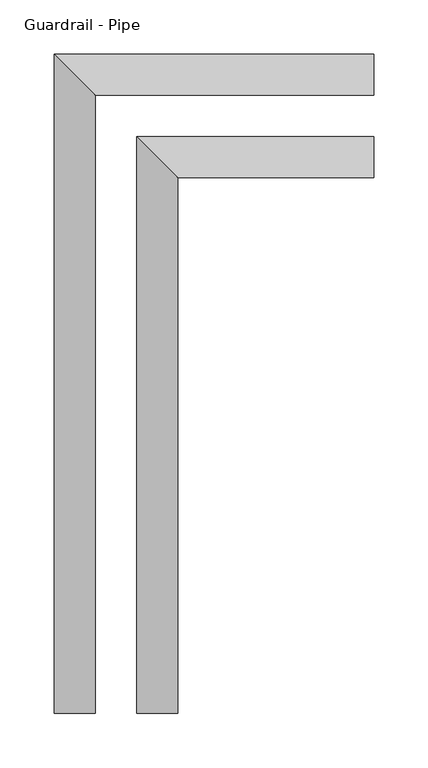
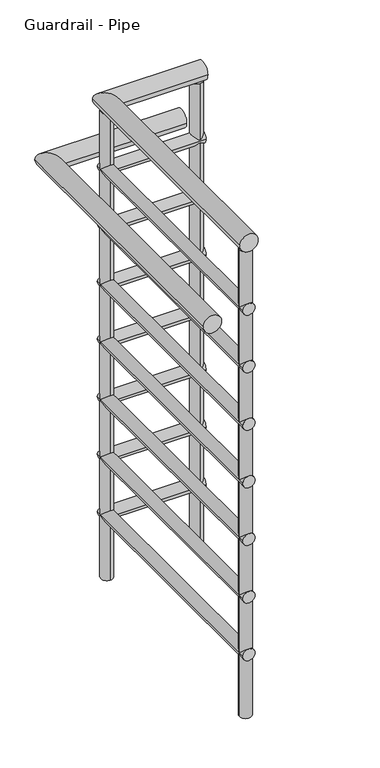
"""IFC4 building model written with IfcOpenShell, lengths in millimetres: railing geometry, Guardrail - Pipe."""

from ifc_helpers import new_model, si_unit, point, frame, frame_2d, origin, place, context, project, spatial, circle_curve, ellipse_curve, trimmed, segment, composite_curve, outline, extrude, source, transform, mapped, element, save
from ifc_brep_helpers import plane_surface, cylinder_surface, advanced_brep


def guardrail_pipe_7d06cf3b(model_context):
    return source(origin(), model_context, "Body", "SolidModel", [
        advanced_brep(
        [(-10864.1022358, -5457.4797826, 4705.35), (-10826.0022358, -5457.4797826, 4705.35), (-10864.1022358, -4924.0797826, 4705.35), (-10826.0022358, -4962.1797826, 4705.35), (-10645.1029016, -4924.0797826, 4705.35), (-10645.1029016, -4962.1797826, 4705.35)],
        [
            (0, 1, circle_curve(frame((-10845.0522358, -5457.4797826, 4705.35), z_axis=(0.0, -1.0, 0.0), x_axis=(1.0, 0.0, 0.0)), 19.05)),
            (1, 0, circle_curve(frame((-10845.0522358, -5457.4797826, 4705.35), z_axis=(0.0, -1.0, 0.0), x_axis=(1.0, 0.0, 0.0)), 19.05)),
            (2, 3, ellipse_curve(frame((-10845.0522358, -4943.1297826, 4705.35), z_axis=(-0.7071067811865502, -0.7071067811865449, 0.0), x_axis=(-0.707106781186545, 0.70710678118655, 0.0)), 26.9407684, 19.05)),
            (3, 1),
            (0, 2),
            (3, 2, ellipse_curve(frame((-10845.0522358, -4943.1297826, 4705.35), z_axis=(-0.7071067811865502, -0.7071067811865449, 0.0), x_axis=(-0.707106781186545, 0.70710678118655, 0.0)), 26.9407684, 19.05)),
            (4, 5, circle_curve(frame((-10645.1029016, -4943.1297826, 4705.35), z_axis=(1.0, 0.0, 0.0), x_axis=(0.0, -1.0, 0.0)), 19.05)),
            (5, 4, circle_curve(frame((-10645.1029016, -4943.1297826, 4705.35), z_axis=(1.0, 0.0, 0.0), x_axis=(0.0, -1.0, 0.0)), 19.05)),
            (5, 3),
            (2, 4),
        ],
        [
            plane_surface(frame((-10845.0522358, -5457.4797826, 4724.4), z_axis=(0.0, -1.0, 0.0), x_axis=(0.0, 0.0, -1.0))),
            cylinder_surface(frame((-10845.0522358, -4943.1297826, 4705.35), z_axis=(0.0, 1.0, 0.0), x_axis=(1.0, 0.0, 0.0)), 19.05),
            plane_surface(frame((-10645.1029016, -4943.1297826, 4724.4), z_axis=(1.0, 0.0, 0.0), x_axis=(0.0, -1.0, 0.0))),
            cylinder_surface(frame((-10645.1029016, -4943.1297826, 4705.35), z_axis=(1.0, 0.0, 0.0), x_axis=(0.0, -1.0, 0.0)), 19.05),
        ],
        [
            (0, [[1, 2]]),
            (1, [[3, 4, -1, 5]]),
            (1, [[6, -5, -2, -4]]),
            (2, [[7, 8]]),
            (3, [[-8, 9, -3, 10]]),
            (3, [[-7, -10, -6, -9]]),
        ],
    ),
        advanced_brep(
        [(-10645.1029016, -4930.4297826, 4559.3), (-10645.1029016, -4955.8297826, 4559.3), (-10832.3522358, -4955.8297826, 4559.3), (-10857.7522358, -4930.4297826, 4559.3), (-10857.7522358, -5457.4797826, 4559.3), (-10832.3522358, -5457.4797826, 4559.3)],
        [
            (0, 1, circle_curve(frame((-10645.1029016, -4943.1297826, 4559.3), z_axis=(1.0, 0.0, 0.0), x_axis=(0.0, -1.0, 0.0)), 12.7)),
            (1, 0, circle_curve(frame((-10645.1029016, -4943.1297826, 4559.3), z_axis=(1.0, 0.0, 0.0), x_axis=(0.0, -1.0, 0.0)), 12.7)),
            (1, 2),
            (2, 3, ellipse_curve(frame((-10845.0522358, -4943.1297826, 4559.3), z_axis=(0.7071067811865502, 0.7071067811865449, 0.0), x_axis=(0.7071067811865447, -0.7071067811865503, 0.0)), 17.9605122, 12.7)),
            (3, 0),
            (3, 2, ellipse_curve(frame((-10845.0522358, -4943.1297826, 4559.3), z_axis=(0.7071067811865502, 0.7071067811865449, 0.0), x_axis=(0.7071067811865447, -0.7071067811865503, 0.0)), 17.9605122, 12.7)),
            (4, 5, circle_curve(frame((-10845.0522358, -5457.4797826, 4559.3), z_axis=(0.0, -1.0, 0.0), x_axis=(1.0, 0.0, 0.0)), 12.7)),
            (5, 4, circle_curve(frame((-10845.0522358, -5457.4797826, 4559.3), z_axis=(0.0, -1.0, 0.0), x_axis=(1.0, 0.0, 0.0)), 12.7)),
            (2, 5),
            (4, 3),
        ],
        [
            plane_surface(frame((-10645.1029016, -4943.1297826, 4572.0), z_axis=(1.0, 0.0, 0.0), x_axis=(0.0, -1.0, 0.0))),
            cylinder_surface(frame((-10645.1029016, -4943.1297826, 4559.3), z_axis=(1.0, 0.0, 0.0), x_axis=(0.0, -1.0, 0.0)), 12.7),
            plane_surface(frame((-10845.0522358, -5457.4797826, 4572.0), z_axis=(0.0, -1.0, 0.0), x_axis=(0.0, 0.0, -1.0))),
            cylinder_surface(frame((-10845.0522358, -4943.1297826, 4559.3), z_axis=(0.0, 1.0, 0.0), x_axis=(1.0, 0.0, 0.0)), 12.7),
        ],
        [
            (0, [[1, 2]]),
            (1, [[-2, 3, 4, 5]]),
            (1, [[-1, -5, 6, -3]]),
            (2, [[7, 8]]),
            (3, [[-4, 9, -7, 10]]),
            (3, [[-6, -10, -8, -9]]),
        ],
    ),
        advanced_brep(
        [(-10940.3022358, -5457.4797826, 4552.95), (-10902.2022358, -5457.4797826, 4552.95), (-10940.3022358, -4847.8797826, 4552.95), (-10902.2022358, -4885.9797826, 4552.95), (-10645.1029016, -4847.8797826, 4552.95), (-10645.1029016, -4885.9797826, 4552.95)],
        [
            (0, 1, circle_curve(frame((-10921.2522358, -5457.4797826, 4552.95), z_axis=(0.0, -1.0, 0.0), x_axis=(1.0, 0.0, 0.0)), 19.05)),
            (1, 0, circle_curve(frame((-10921.2522358, -5457.4797826, 4552.95), z_axis=(0.0, -1.0, 0.0), x_axis=(1.0, 0.0, 0.0)), 19.05)),
            (2, 3, ellipse_curve(frame((-10921.2522358, -4866.9297826, 4552.95), z_axis=(-0.7071067811865502, -0.7071067811865449, 0.0), x_axis=(-0.707106781186545, 0.70710678118655, 0.0)), 26.9407684, 19.05)),
            (3, 1),
            (0, 2),
            (3, 2, ellipse_curve(frame((-10921.2522358, -4866.9297826, 4552.95), z_axis=(-0.7071067811865502, -0.7071067811865449, 0.0), x_axis=(-0.707106781186545, 0.70710678118655, 0.0)), 26.9407684, 19.05)),
            (4, 5, circle_curve(frame((-10645.1029016, -4866.9297826, 4552.95), z_axis=(1.0, 0.0, 0.0), x_axis=(0.0, -1.0, 0.0)), 19.05)),
            (5, 4, circle_curve(frame((-10645.1029016, -4866.9297826, 4552.95), z_axis=(1.0, 0.0, 0.0), x_axis=(0.0, -1.0, 0.0)), 19.05)),
            (4, 2),
            (3, 5),
        ],
        [
            plane_surface(frame((-10921.2522358, -5457.4797826, 4572.0), z_axis=(0.0, -1.0, 0.0), x_axis=(0.0, 0.0, -1.0))),
            cylinder_surface(frame((-10921.2522358, -4866.9297826, 4552.95), z_axis=(0.0, 1.0, 0.0), x_axis=(1.0, 0.0, 0.0)), 19.05),
            plane_surface(frame((-10645.1029016, -4866.9297826, 4572.0), z_axis=(1.0, 0.0, 0.0), x_axis=(0.0, -1.0, 0.0))),
            cylinder_surface(frame((-10645.1029016, -4866.9297826, 4552.95), z_axis=(1.0, 0.0, 0.0), x_axis=(0.0, -1.0, 0.0)), 19.05),
        ],
        [
            (0, [[1, 2]]),
            (1, [[3, 4, -1, 5]]),
            (1, [[6, -5, -2, -4]]),
            (2, [[7, 8]]),
            (3, [[-7, 9, -6, 10]]),
            (3, [[-8, -10, -3, -9]]),
        ],
    ),
        advanced_brep(
        [(-10645.1029016, -4930.4297826, 4432.3), (-10645.1029016, -4955.8297826, 4432.3), (-10832.3522358, -4955.8297826, 4432.3), (-10857.7522358, -4930.4297826, 4432.3), (-10857.7522358, -5457.4797826, 4432.3), (-10832.3522358, -5457.4797826, 4432.3)],
        [
            (0, 1, circle_curve(frame((-10645.1029016, -4943.1297826, 4432.3), z_axis=(1.0, 0.0, 0.0), x_axis=(0.0, -1.0, 0.0)), 12.7)),
            (1, 0, circle_curve(frame((-10645.1029016, -4943.1297826, 4432.3), z_axis=(1.0, 0.0, 0.0), x_axis=(0.0, -1.0, 0.0)), 12.7)),
            (1, 2),
            (2, 3, ellipse_curve(frame((-10845.0522358, -4943.1297826, 4432.3), z_axis=(0.7071067811865502, 0.7071067811865449, 0.0), x_axis=(0.7071067811865447, -0.7071067811865503, 0.0)), 17.9605122, 12.7)),
            (3, 0),
            (3, 2, ellipse_curve(frame((-10845.0522358, -4943.1297826, 4432.3), z_axis=(0.7071067811865502, 0.7071067811865449, 0.0), x_axis=(0.7071067811865447, -0.7071067811865503, 0.0)), 17.9605122, 12.7)),
            (4, 5, circle_curve(frame((-10845.0522358, -5457.4797826, 4432.3), z_axis=(0.0, -1.0, 0.0), x_axis=(1.0, 0.0, 0.0)), 12.7)),
            (5, 4, circle_curve(frame((-10845.0522358, -5457.4797826, 4432.3), z_axis=(0.0, -1.0, 0.0), x_axis=(1.0, 0.0, 0.0)), 12.7)),
            (2, 5),
            (4, 3),
        ],
        [
            plane_surface(frame((-10645.1029016, -4943.1297826, 4445.0), z_axis=(1.0, 0.0, 0.0), x_axis=(0.0, -1.0, 0.0))),
            cylinder_surface(frame((-10645.1029016, -4943.1297826, 4432.3), z_axis=(1.0, 0.0, 0.0), x_axis=(0.0, -1.0, 0.0)), 12.7),
            plane_surface(frame((-10845.0522358, -5457.4797826, 4445.0), z_axis=(0.0, -1.0, 0.0), x_axis=(0.0, 0.0, -1.0))),
            cylinder_surface(frame((-10845.0522358, -4943.1297826, 4432.3), z_axis=(0.0, 1.0, 0.0), x_axis=(1.0, 0.0, 0.0)), 12.7),
        ],
        [
            (0, [[1, 2]]),
            (1, [[-2, 3, 4, 5]]),
            (1, [[-1, -5, 6, -3]]),
            (2, [[7, 8]]),
            (3, [[-4, 9, -7, 10]]),
            (3, [[-6, -10, -8, -9]]),
        ],
    ),
        advanced_brep(
        [(-10645.1029016, -4930.4297826, 4305.3), (-10645.1029016, -4955.8297826, 4305.3), (-10832.3522358, -4955.8297826, 4305.3), (-10857.7522358, -4930.4297826, 4305.3), (-10857.7522358, -5457.4797826, 4305.3), (-10832.3522358, -5457.4797826, 4305.3)],
        [
            (0, 1, circle_curve(frame((-10645.1029016, -4943.1297826, 4305.3), z_axis=(1.0, 0.0, 0.0), x_axis=(0.0, -1.0, 0.0)), 12.7)),
            (1, 0, circle_curve(frame((-10645.1029016, -4943.1297826, 4305.3), z_axis=(1.0, 0.0, 0.0), x_axis=(0.0, -1.0, 0.0)), 12.7)),
            (1, 2),
            (2, 3, ellipse_curve(frame((-10845.0522358, -4943.1297826, 4305.3), z_axis=(0.7071067811865502, 0.7071067811865449, 0.0), x_axis=(0.7071067811865447, -0.7071067811865503, 0.0)), 17.9605122, 12.7)),
            (3, 0),
            (3, 2, ellipse_curve(frame((-10845.0522358, -4943.1297826, 4305.3), z_axis=(0.7071067811865502, 0.7071067811865449, 0.0), x_axis=(0.7071067811865447, -0.7071067811865503, 0.0)), 17.9605122, 12.7)),
            (4, 5, circle_curve(frame((-10845.0522358, -5457.4797826, 4305.3), z_axis=(0.0, -1.0, 0.0), x_axis=(1.0, 0.0, 0.0)), 12.7)),
            (5, 4, circle_curve(frame((-10845.0522358, -5457.4797826, 4305.3), z_axis=(0.0, -1.0, 0.0), x_axis=(1.0, 0.0, 0.0)), 12.7)),
            (2, 5),
            (4, 3),
        ],
        [
            plane_surface(frame((-10645.1029016, -4943.1297826, 4318.0), z_axis=(1.0, 0.0, 0.0), x_axis=(0.0, -1.0, 0.0))),
            cylinder_surface(frame((-10645.1029016, -4943.1297826, 4305.3), z_axis=(1.0, 0.0, 0.0), x_axis=(0.0, -1.0, 0.0)), 12.7),
            plane_surface(frame((-10845.0522358, -5457.4797826, 4318.0), z_axis=(0.0, -1.0, 0.0), x_axis=(0.0, 0.0, -1.0))),
            cylinder_surface(frame((-10845.0522358, -4943.1297826, 4305.3), z_axis=(0.0, 1.0, 0.0), x_axis=(1.0, 0.0, 0.0)), 12.7),
        ],
        [
            (0, [[1, 2]]),
            (1, [[-2, 3, 4, 5]]),
            (1, [[-1, -5, 6, -3]]),
            (2, [[7, 8]]),
            (3, [[-4, 9, -7, 10]]),
            (3, [[-6, -10, -8, -9]]),
        ],
    ),
        advanced_brep(
        [(-10645.1029016, -4930.4297826, 4178.3), (-10645.1029016, -4955.8297826, 4178.3), (-10832.3522358, -4955.8297826, 4178.3), (-10857.7522358, -4930.4297826, 4178.3), (-10857.7522358, -5457.4797826, 4178.3), (-10832.3522358, -5457.4797826, 4178.3)],
        [
            (0, 1, circle_curve(frame((-10645.1029016, -4943.1297826, 4178.3), z_axis=(1.0, 0.0, 0.0), x_axis=(0.0, -1.0, 0.0)), 12.7)),
            (1, 0, circle_curve(frame((-10645.1029016, -4943.1297826, 4178.3), z_axis=(1.0, 0.0, 0.0), x_axis=(0.0, -1.0, 0.0)), 12.7)),
            (1, 2),
            (2, 3, ellipse_curve(frame((-10845.0522358, -4943.1297826, 4178.3), z_axis=(0.7071067811865502, 0.7071067811865449, 0.0), x_axis=(0.7071067811865447, -0.7071067811865503, 0.0)), 17.9605122, 12.7)),
            (3, 0),
            (3, 2, ellipse_curve(frame((-10845.0522358, -4943.1297826, 4178.3), z_axis=(0.7071067811865502, 0.7071067811865449, 0.0), x_axis=(0.7071067811865447, -0.7071067811865503, 0.0)), 17.9605122, 12.7)),
            (4, 5, circle_curve(frame((-10845.0522358, -5457.4797826, 4178.3), z_axis=(0.0, -1.0, 0.0), x_axis=(1.0, 0.0, 0.0)), 12.7)),
            (5, 4, circle_curve(frame((-10845.0522358, -5457.4797826, 4178.3), z_axis=(0.0, -1.0, 0.0), x_axis=(1.0, 0.0, 0.0)), 12.7)),
            (2, 5),
            (4, 3),
        ],
        [
            plane_surface(frame((-10645.1029016, -4943.1297826, 4191.0), z_axis=(1.0, 0.0, 0.0), x_axis=(0.0, -1.0, 0.0))),
            cylinder_surface(frame((-10645.1029016, -4943.1297826, 4178.3), z_axis=(1.0, 0.0, 0.0), x_axis=(0.0, -1.0, 0.0)), 12.7),
            plane_surface(frame((-10845.0522358, -5457.4797826, 4191.0), z_axis=(0.0, -1.0, 0.0), x_axis=(0.0, 0.0, -1.0))),
            cylinder_surface(frame((-10845.0522358, -4943.1297826, 4178.3), z_axis=(0.0, 1.0, 0.0), x_axis=(1.0, 0.0, 0.0)), 12.7),
        ],
        [
            (0, [[1, 2]]),
            (1, [[-2, 3, 4, 5]]),
            (1, [[-1, -5, 6, -3]]),
            (2, [[7, 8]]),
            (3, [[-4, 9, -7, 10]]),
            (3, [[-6, -10, -8, -9]]),
        ],
    ),
        advanced_brep(
        [(-10645.1029016, -4930.4297826, 4051.3), (-10645.1029016, -4955.8297826, 4051.3), (-10832.3522358, -4955.8297826, 4051.3), (-10857.7522358, -4930.4297826, 4051.3), (-10857.7522358, -5457.4797826, 4051.3), (-10832.3522358, -5457.4797826, 4051.3)],
        [
            (0, 1, circle_curve(frame((-10645.1029016, -4943.1297826, 4051.3), z_axis=(1.0, 0.0, 0.0), x_axis=(0.0, -1.0, 0.0)), 12.7)),
            (1, 0, circle_curve(frame((-10645.1029016, -4943.1297826, 4051.3), z_axis=(1.0, 0.0, 0.0), x_axis=(0.0, -1.0, 0.0)), 12.7)),
            (1, 2),
            (2, 3, ellipse_curve(frame((-10845.0522358, -4943.1297826, 4051.3), z_axis=(0.7071067811865502, 0.7071067811865449, 0.0), x_axis=(0.7071067811865447, -0.7071067811865503, 0.0)), 17.9605122, 12.7)),
            (3, 0),
            (3, 2, ellipse_curve(frame((-10845.0522358, -4943.1297826, 4051.3), z_axis=(0.7071067811865502, 0.7071067811865449, 0.0), x_axis=(0.7071067811865447, -0.7071067811865503, 0.0)), 17.9605122, 12.7)),
            (4, 5, circle_curve(frame((-10845.0522358, -5457.4797826, 4051.3), z_axis=(0.0, -1.0, 0.0), x_axis=(1.0, 0.0, 0.0)), 12.7)),
            (5, 4, circle_curve(frame((-10845.0522358, -5457.4797826, 4051.3), z_axis=(0.0, -1.0, 0.0), x_axis=(1.0, 0.0, 0.0)), 12.7)),
            (2, 5),
            (4, 3),
        ],
        [
            plane_surface(frame((-10645.1029016, -4943.1297826, 4064.0), z_axis=(1.0, 0.0, 0.0), x_axis=(0.0, -1.0, 0.0))),
            cylinder_surface(frame((-10645.1029016, -4943.1297826, 4051.3), z_axis=(1.0, 0.0, 0.0), x_axis=(0.0, -1.0, 0.0)), 12.7),
            plane_surface(frame((-10845.0522358, -5457.4797826, 4064.0), z_axis=(0.0, -1.0, 0.0), x_axis=(0.0, 0.0, -1.0))),
            cylinder_surface(frame((-10845.0522358, -4943.1297826, 4051.3), z_axis=(0.0, 1.0, 0.0), x_axis=(1.0, 0.0, 0.0)), 12.7),
        ],
        [
            (0, [[1, 2]]),
            (1, [[-2, 3, 4, 5]]),
            (1, [[-1, -5, 6, -3]]),
            (2, [[7, 8]]),
            (3, [[-4, 9, -7, 10]]),
            (3, [[-6, -10, -8, -9]]),
        ],
    ),
        advanced_brep(
        [(-10645.1029016, -4930.4297826, 3924.3), (-10645.1029016, -4955.8297826, 3924.3), (-10832.3522358, -4955.8297826, 3924.3), (-10857.7522358, -4930.4297826, 3924.3), (-10857.7522358, -5457.4797826, 3924.3), (-10832.3522358, -5457.4797826, 3924.3)],
        [
            (0, 1, circle_curve(frame((-10645.1029016, -4943.1297826, 3924.3), z_axis=(1.0, 0.0, 0.0), x_axis=(0.0, -1.0, 0.0)), 12.7)),
            (1, 0, circle_curve(frame((-10645.1029016, -4943.1297826, 3924.3), z_axis=(1.0, 0.0, 0.0), x_axis=(0.0, -1.0, 0.0)), 12.7)),
            (1, 2),
            (2, 3, ellipse_curve(frame((-10845.0522358, -4943.1297826, 3924.3), z_axis=(0.7071067811865502, 0.7071067811865449, 0.0), x_axis=(0.7071067811865447, -0.7071067811865503, 0.0)), 17.9605122, 12.7)),
            (3, 0),
            (3, 2, ellipse_curve(frame((-10845.0522358, -4943.1297826, 3924.3), z_axis=(0.7071067811865502, 0.7071067811865449, 0.0), x_axis=(0.7071067811865447, -0.7071067811865503, 0.0)), 17.9605122, 12.7)),
            (4, 5, circle_curve(frame((-10845.0522358, -5457.4797826, 3924.3), z_axis=(0.0, -1.0, 0.0), x_axis=(1.0, 0.0, 0.0)), 12.7)),
            (5, 4, circle_curve(frame((-10845.0522358, -5457.4797826, 3924.3), z_axis=(0.0, -1.0, 0.0), x_axis=(1.0, 0.0, 0.0)), 12.7)),
            (2, 5),
            (4, 3),
        ],
        [
            plane_surface(frame((-10645.1029016, -4943.1297826, 3937.0), z_axis=(1.0, 0.0, 0.0), x_axis=(0.0, -1.0, 0.0))),
            cylinder_surface(frame((-10645.1029016, -4943.1297826, 3924.3), z_axis=(1.0, 0.0, 0.0), x_axis=(0.0, -1.0, 0.0)), 12.7),
            plane_surface(frame((-10845.0522358, -5457.4797826, 3937.0), z_axis=(0.0, -1.0, 0.0), x_axis=(0.0, 0.0, -1.0))),
            cylinder_surface(frame((-10845.0522358, -4943.1297826, 3924.3), z_axis=(0.0, 1.0, 0.0), x_axis=(1.0, 0.0, 0.0)), 12.7),
        ],
        [
            (0, [[1, 2]]),
            (1, [[-2, 3, 4, 5]]),
            (1, [[-1, -5, 6, -3]]),
            (2, [[7, 8]]),
            (3, [[-4, 9, -7, 10]]),
            (3, [[-6, -10, -8, -9]]),
        ],
    ),
        advanced_brep(
        [(-10645.1029016, -4930.4297826, 3797.3), (-10645.1029016, -4955.8297826, 3797.3), (-10832.3522358, -4955.8297826, 3797.3), (-10857.7522358, -4930.4297826, 3797.3), (-10857.7522358, -5457.4797826, 3797.3), (-10832.3522358, -5457.4797826, 3797.3)],
        [
            (0, 1, circle_curve(frame((-10645.1029016, -4943.1297826, 3797.3), z_axis=(1.0, 0.0, 0.0), x_axis=(0.0, -1.0, 0.0)), 12.7)),
            (1, 0, circle_curve(frame((-10645.1029016, -4943.1297826, 3797.3), z_axis=(1.0, 0.0, 0.0), x_axis=(0.0, -1.0, 0.0)), 12.7)),
            (1, 2),
            (2, 3, ellipse_curve(frame((-10845.0522358, -4943.1297826, 3797.3), z_axis=(0.7071067811865502, 0.7071067811865449, 0.0), x_axis=(0.7071067811865447, -0.7071067811865503, 0.0)), 17.9605122, 12.7)),
            (3, 0),
            (3, 2, ellipse_curve(frame((-10845.0522358, -4943.1297826, 3797.3), z_axis=(0.7071067811865502, 0.7071067811865449, 0.0), x_axis=(0.7071067811865447, -0.7071067811865503, 0.0)), 17.9605122, 12.7)),
            (4, 5, circle_curve(frame((-10845.0522358, -5457.4797826, 3797.3), z_axis=(0.0, -1.0, 0.0), x_axis=(1.0, 0.0, 0.0)), 12.7)),
            (5, 4, circle_curve(frame((-10845.0522358, -5457.4797826, 3797.3), z_axis=(0.0, -1.0, 0.0), x_axis=(1.0, 0.0, 0.0)), 12.7)),
            (2, 5),
            (4, 3),
        ],
        [
            plane_surface(frame((-10645.1029016, -4943.1297826, 3810.0), z_axis=(1.0, 0.0, 0.0), x_axis=(0.0, -1.0, 0.0))),
            cylinder_surface(frame((-10645.1029016, -4943.1297826, 3797.3), z_axis=(1.0, 0.0, 0.0), x_axis=(0.0, -1.0, 0.0)), 12.7),
            plane_surface(frame((-10845.0522358, -5457.4797826, 3810.0), z_axis=(0.0, -1.0, 0.0), x_axis=(0.0, 0.0, -1.0))),
            cylinder_surface(frame((-10845.0522358, -4943.1297826, 3797.3), z_axis=(0.0, 1.0, 0.0), x_axis=(1.0, 0.0, 0.0)), 12.7),
        ],
        [
            (0, [[1, 2]]),
            (1, [[-2, 3, 4, 5]]),
            (1, [[-1, -5, 6, -3]]),
            (2, [[7, 8]]),
            (3, [[-4, 9, -7, 10]]),
            (3, [[-6, -10, -8, -9]]),
        ],
    ),
        extrude(outline(composite_curve([segment(trimmed(circle_curve(frame_2d((-10845.0522358, -4943.1297826)), 12.7), [point((-10845.0522358, -4930.4297826))], [point((-10845.0522358, -4955.8297826))], False, "CARTESIAN"), True, "CONTINUOUS"), segment(trimmed(circle_curve(frame_2d((-10845.0522358, -4943.1297826)), 12.7), [point((-10845.0522358, -4955.8297826))], [point((-10845.0522358, -4930.4297826))], False, "CARTESIAN"), True, "CONTINUOUS")], self_intersect=False)), frame((0.0, 0.0, 3657.6), z_axis=(0.0, 0.0, 1.0), x_axis=(1.0, 0.0, 0.0)), (0.0, 0.0, 1.0), 1028.7),
        extrude(outline(composite_curve([segment(trimmed(circle_curve(frame_2d((-10845.0522358, -5444.7797826)), 12.7), [point((-10857.7522358, -5444.7797826))], [point((-10832.3522358, -5444.7797826))], False, "CARTESIAN"), True, "CONTINUOUS"), segment(trimmed(circle_curve(frame_2d((-10845.0522358, -5444.7797826)), 12.7), [point((-10832.3522358, -5444.7797826))], [point((-10857.7522358, -5444.7797826))], False, "CARTESIAN"), True, "CONTINUOUS")], self_intersect=False)), frame((0.0, 0.0, 3657.6), z_axis=(0.0, 0.0, 1.0), x_axis=(1.0, 0.0, 0.0)), (0.0, 0.0, 1.0), 1028.7),
        extrude(outline(composite_curve([segment(trimmed(circle_curve(frame_2d((-10657.8029016, -4943.1297826)), 12.7), [point((-10657.8029016, -4930.4297826))], [point((-10657.8029016, -4955.8297826))], False, "CARTESIAN"), True, "CONTINUOUS"), segment(trimmed(circle_curve(frame_2d((-10657.8029016, -4943.1297826)), 12.7), [point((-10657.8029016, -4955.8297826))], [point((-10657.8029016, -4930.4297826))], False, "CARTESIAN"), True, "CONTINUOUS")], self_intersect=False)), frame((0.0, 0.0, 3657.6), z_axis=(0.0, 0.0, 1.0), x_axis=(1.0, 0.0, 0.0)), (0.0, 0.0, 1.0), 1028.7),
    ])


if __name__ == "__main__":
    model = new_model("IFC4")
    model_context = context("Model", 3, world=origin())
    ifc_project = project(units=[si_unit("LENGTHUNIT", "METRE", prefix="MILLI")], contexts=[model_context])
    site = spatial("IfcSite", under=ifc_project)
    building = spatial("IfcBuilding", under=site)
    placement = place(None, origin())
    guardrail_pipe_shape = guardrail_pipe_7d06cf3b(model_context)
    element("IfcRailing", 1, ObjectType="Guardrail - Pipe", at=placement, inside=building, context=model_context, shape_type="MappedRepresentation", body=[
        mapped(guardrail_pipe_shape, transform((0.0, 0.0, 0.0), x_axis=(1.0, 0.0, 0.0), y_axis=(0.0, 1.0, 0.0), z_axis=(0.0, 0.0, 1.0))),
    ])
    save(model, "model.ifc")

# Revit data of these elements
# Element 1 (IfcRailing, "Guardrail - Pipe")
#   Materials on its faces: "Plastic - Vinyl Cove Base"
# Materials
#   "Plastic - Vinyl Cove Base": class "Plastic", colour RGB 5 5 5, transparency 0, Cost = 0
